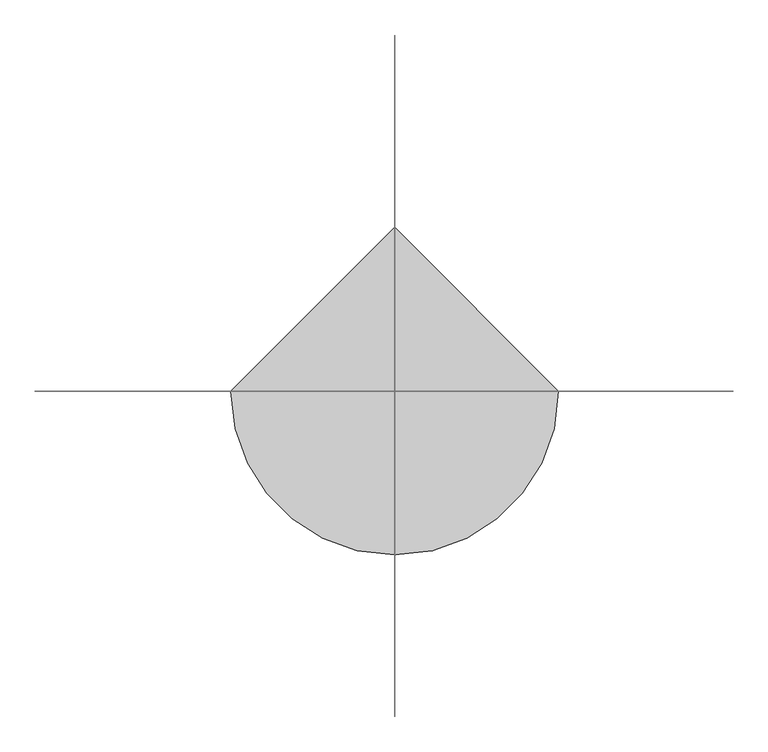
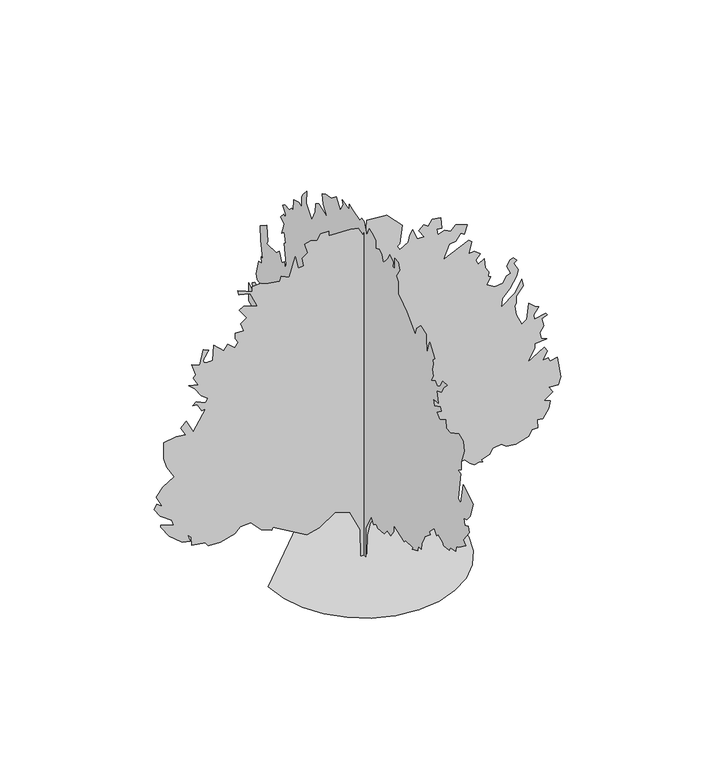
"""IFC4 building model written with IfcOpenShell, lengths in millimetres: proxy geometry, daphne 26070 : daphne 26070."""

from ifc_helpers import new_model, si_unit, origin, place, context, project, spatial, triangles, source, transform, mapped, element, save


def entourage_7462b660(model_context):
    return source(origin(), model_context, "Body", "Tessellation", [
        triangles([(-9.4573925, -3.9e-06, 72.2348623), (-36.4693492, -6.1e-06, 128.8771626), (-74.629579, -5.2e-06, 141.2324949), (-113.9485589, -1.8e-06, 114.0498972), (-145.9624841, 1e-07, 106.0463523), (-234.001251, 8e-07, 158.0691489), (-236.002001, 1.4e-06, 150.0658583), (-264.0154255, 1.9e-06, 162.0709213), (-290.0250479, 1.3e-06, 190.0833467), (-318.0387268, 2.7e-06, 188.0823242), (-332.0443036, 4.1e-06, 174.0762387), (-368.4272936, 6.4e-06, 163.6409018), (-400.0731817, 7.6e-06, 166.0726938), (-408.0767266, 7.3e-06, 176.0772612), (-442.0924192, 8.5e-06, 182.0797836), (-444.0939686, 7.2e-06, 204.089414), (-452.0975135, 7.1e-06, 212.0929589), (-446.0929381, 7.9e-06, 194.0851191), (-466.1030903, 8.6e-06, 198.0868916), (-500.1187829, 8.4e-06, 226.0990444), (-522.1279046, 7.4e-06, 258.1124609), (-522.1279046, 7.1e-06, 264.1170363), (-488.1121757, 6.3e-06, 252.1104472), (-494.1142076, 5.6e-06, 268.117537), (-522.9229142, 5.6e-06, 288.9353979), (-538.1349944, 4.9e-06, 312.1357804), (-532.1304191, 3.9e-06, 324.1423513), (-518.1248423, 3.9e-06, 314.1372934), (-534.1319321, 2.8e-06, 344.14996), (-516.6084741, 8e-07, 365.2878413), (-486.7989927, -1.6e-06, 383.4742676), (-506.1208148, -2.7e-06, 416.1818642), (-514.1243597, -3.9e-06, 442.1940482), (-514.1243597, -6.5e-06, 486.2122553), (-482.1101801, -8.1e-06, 490.2153176), (-458.099509, -9.1e-06, 488.2138046), (-470.1035728, -9.9e-06, 510.2229263), (-456.097996, -1.13e-05, 524.2284668), (-438.0893932, -1e-05, 488.2138046), (-406.0752136, -1.45e-05, 540.2355566), (-416.0802715, -1.39e-05, 538.236587), (-428.0868788, -1.46e-05, 558.2441957), (-440.0909062, -1.42e-05, 560.2457088), (-430.0883918, -1.51e-05, 568.2492537), (-406.0752136, -1.54e-05, 556.2426827), (-401.4955876, -1.62e-05, 567.0275259), (-418.0817845, -1.63e-05, 580.2533175), (-434.0888743, -1.7e-05, 604.2639522), (-450.0959641, -1.72e-05, 618.2720724), (-426.0853294, -1.79e-05, 612.2674971), (-438.0893932, -1.87e-05, 634.2791622), (-432.0873613, -1.94e-05, 642.2826708), (-442.0924192, -2.07e-05, 672.2953737), (-422.0823034, -2.11e-05, 664.2917925), (-412.0797526, -2.38e-05, 702.308004), (-398.0716687, -2.41e-05, 696.3059721), (-400.6802304, -2.38e-05, 693.2783226), (-403.212634, -2.35e-05, 690.2023476), (-405.5926123, -2.32e-05, 687.0248526), (-407.7439708, -2.29e-05, 683.6948959), (-409.5930948, -2.26e-05, 680.1642975), (-411.0637536, -2.23e-05, 676.3821882), (-412.0797526, -2.21e-05, 672.2953737), (-411.9857903, -2.19e-05, 668.7317104), (-410.3525688, -2.18e-05, 666.420369), (-407.434106, -2.18e-05, 665.1452288), (-403.4920137, -2.2e-05, 664.7033226), (-398.7777666, -2.22e-05, 664.8861603), (-393.5530128, -2.25e-05, 665.485615), (-388.0691179, -2.28e-05, 666.2907984), (-386.0676049, -2.52e-05, 706.3085592), (-360.0554572, -2.49e-05, 682.2978882), (-350.0529064, -2.62e-05, 696.3059721), (-332.0443036, -2.6e-05, 680.2988823), (-322.0392457, -2.72e-05, 692.3029461), (-330.0427906, -2.76e-05, 704.3095533), (-330.0427906, -2.84e-05, 718.3150938), (-308.0336689, -2.94e-05, 718.3150938), (-316.0372138, -3.03e-05, 740.3242155), (-301.0029389, -3.16e-05, 751.5637184), (-320.0377327, -3.24e-05, 778.340427), (-308.0336689, -3.33e-05, 784.3424589), (-274.0179581, -3.42e-05, 774.3399445), (-292.0265791, -3.57e-05, 812.356156), (-320.9191106, -3.49e-05, 820.7254852), (-324.0407587, -3.54e-05, 832.3637283), (-304.0306247, -3.58e-05, 824.3602198), (-286.0245472, -3.62e-05, 816.3566385), (-286.0245472, -3.7e-05, 830.3647951), (-265.0619096, -3.8e-05, 832.6329706), (-252.0090908, -3.82e-05, 826.3616964), (-215.9931387, -3.95e-05, 820.3596645), (-211.9913662, -4.03e-05, 832.3637283), (-191.9827583, -4.06e-05, 822.3612139), (-175.9756504, -4.43e-05, 872.3814892), (-168.7203883, -4.27e-05, 839.3385933), (-153.9660381, -4.34e-05, 840.3673096), (-157.9678106, -4.45e-05, 862.3789747), (-143.9617251, -4.57e-05, 872.3814892), (-151.9650156, -4.69e-05, 898.3936369), (-135.9581802, -4.78e-05, 902.3941195), (-119.9513447, -4.83e-05, 898.3936369), (-109.9467864, -4.96e-05, 912.3991774), (-89.9381694, -5.05e-05, 912.3991774), (-89.9381694, -4.97e-05, 900.3951862), (-32.626833, -5.21e-05, 897.7739073), (-14.3439498, -5.26e-05, 893.5625364), (-1.8993678, -5.19e-05, 872.3814892), (6.1041838, -5.31e-05, 886.3895731), (8.105045, -5.45e-05, 908.3986948), (59.627565, -5.65e-05, 903.8140182), (99.4230465, -5.58e-05, 862.5999641), (92.1418776, -5.26e-05, 814.3577053), (86.1393461, -5.21e-05, 810.3546066), (92.1418776, -5.16e-05, 798.3505428), (114.1514989, -5.33e-05, 810.3546066), (118.1578496, -5.45e-05, 827.9416145), (126.1568253, -5.56e-05, 840.3673096), (138.1621427, -5.45e-05, 812.356156), (155.7905089, -5.52e-05, 811.8684677), (142.1639151, -5.58e-05, 832.3637283), (154.1689872, -5.71e-05, 844.3703356), (166.1743046, -5.71e-05, 836.3667543), (176.1785995, -5.85e-05, 852.3739168), (198.1884842, -5.92e-05, 848.3708181), (200.188998, -5.75e-05, 818.3581879), (188.1839168, -5.71e-05, 820.3596645), (190.1846849, -5.63e-05, 804.3525747), (208.1927972, -5.74e-05, 810.3546066), (224.199887, -5.76e-05, 802.3510981), (236.20495, -5.9e-05, 816.3566385), (265.7807247, -5.96e-05, 805.7293076), (258.2140718, -5.79e-05, 782.343453), (250.2110355, -5.79e-05, 788.3454849), (236.20495, -5.62e-05, 770.3369184), (220.1978602, -5.54e-05, 768.3379126), (204.1910248, -5.26e-05, 732.3207069), (270.2206608, -5.73e-05, 762.3333372), (278.2242057, -5.71e-05, 754.3298286), (270.2206608, -5.5e-05, 724.3171257), (284.2262195, -5.57e-05, 726.318675), (300.2333274, -5.57e-05, 714.3120678), (288.2267384, -5.43e-05, 700.3065273), (294.2312955, -5.39e-05, 688.3024635), (309.737998, -5.51e-05, 697.179756), (312.8444218, -5.37e-05, 671.3504459), (322.242431, -5.33e-05, 658.2872171), (320.240918, -5.25e-05, 646.283226), (326.2454933, -5.25e-05, 642.2801273), (316.2403991, -5.1e-05, 624.2741043), (337.7847236, -5.12e-05, 610.9797123), (358.2596729, -5.23e-05, 614.2690464), (368.2621874, -5.37e-05, 630.2761362), (378.0386619, -5.44e-05, 634.7135107), (368.2621874, -5.52e-05, 656.2882839), (376.2657323, -5.64e-05, 670.2938244), (384.2692772, -5.7e-05, 674.2943069), (394.2743714, -5.68e-05, 664.2917925), (386.2708265, -5.61e-05, 658.2872171), (398.1707179, -5.54e-05, 637.1290609), (394.2743714, -5.43e-05, 622.272555), (376.2657323, -5.17e-05, 592.2598884), (356.2581599, -4.97e-05, 572.2497725), (354.2566106, -4.83e-05, 550.2406508), (388.2723395, -5.13e-05, 576.2527986), (406.2783989, -5.4e-05, 608.2669782), (410.2814612, -5.3e-05, 588.2568624), (392.2728221, -5.09e-05, 566.2477407), (392.2728221, -4.98e-05, 548.2391015), (388.2723395, -4.93e-05, 542.2371059), (392.2728221, -4.79e-05, 516.2249219), (406.2783989, -4.67e-05, 486.2122553), (419.6692966, -4.79e-05, 495.1530613), (424.2870017, -5.05e-05, 536.235074), (440.2941278, -5.04e-05, 522.2294972), (450.2991858, -5.06e-05, 518.2264712), (437.047996, -4.89e-05, 500.1924339), (438.2925785, -4.83e-05, 488.2138046), (468.3077886, -4.99e-05, 494.2158002), (472.3083075, -4.97e-05, 488.2138046), (458.3027307, -4.88e-05, 482.2117727), (462.5902596, -4.78e-05, 462.3895815), (452.3006988, -4.64e-05, 446.1945308), (456.3012177, -4.56e-05, 430.187441), (470.3067581, -4.58e-05, 424.1854091), (440.2941278, -4.43e-05, 420.1849265), (440.2941278, -4.36e-05, 408.1783193), (420.2865191, -4.08e-05, 376.1641397), (464.3047626, -4.43e-05, 402.1762874), (472.3083075, -4.39e-05, 390.1697165), (460.3017002, -4.21e-05, 368.1605947), (474.3098205, -4.28e-05, 370.1621078), (478.3103394, -4.24e-05, 360.1570498), (498.3204552, -4.35e-05, 364.1600759), (506.3240001, -4.05e-05, 308.1352615), (500.3194247, -3.9e-05, 288.1251276), (476.3113335, -3.81e-05, 290.1266587), (486.3138843, -3.76e-05, 274.1195508), (464.3047626, -3.57e-05, 258.1124609), (480.3118524, -3.6e-05, 252.1104472), (476.3113335, -3.47e-05, 232.1015668), (460.3017002, -3.26e-05, 210.0919546), (446.2961234, -3.22e-05, 212.0929589), (448.2976727, -3.09e-05, 190.0833467), (432.2905829, -3.02e-05, 190.0833467), (424.2870017, -2.89e-05, 174.0762387), (391.7419679, -2.69e-05, 164.3614974), (366.2632178, -2.6e-05, 168.0737163), (354.2566106, -2.61e-05, 178.0780111), (332.2474889, -2.49e-05, 174.0762387), (323.8020015, -2.37e-05, 160.8723026), (302.2348404, -2.24e-05, 154.0673764), (306.2353412, -2.21e-05, 146.0640859), (298.2317963, -2.2e-05, 150.0658583), (284.2262195, -2.11e-05, 146.0640859), (272.2196304, -2.11e-05, 154.0673764), (260.2155848, -2.14e-05, 168.0737163), (240.2064682, -2.03e-05, 164.0719438), (236.8051496, -1.96e-05, 155.3752181), (196.1874799, -1.67e-05, 136.0595276), (196.1874799, -1.6e-05, 124.0544646), (162.1725321, -1.36e-05, 110.0481247), (162.1725321, -1.4e-05, 116.0509106), (138.1618883, -1.27e-05, 112.0491381), (106.7192036, -1.23e-05, 127.7984221), (83.214788, -1.13e-05, 128.4156446), (38.7434109, -8e-06, 104.983363), (17.3291135, -5.6e-06, 81.0641653), (9.1189377, -3.5e-06, 51.8726831), (8.1050195, -4e-07, 0.0), (-7.9020227, 3e-07, 7e-07), (-244.9072532, 0.0, 4.54e-05), (-238.4327937, -56.1165193, 4.18e-05), (-219.9933851, -107.6506239, 3.79e-05), (-191.0655541, -153.1257915, 3.39e-05), (-153.1257915, -191.0655541, 3e-05), (-107.6506239, -219.9933851, 2.63e-05), (-56.1165193, -238.4327937, 2.29e-05), (1.14e-05, -244.9072532, 2.01e-05), (56.1165193, -238.4327937, 1.8e-05), (107.6506239, -219.9933851, 5.12e-05), (153.1257915, -191.0655541, 5.1e-05), (191.0655541, -153.1257915, 5.16e-05), (219.9933851, -107.6506239, 1.87e-05), (238.4327937, -56.1165193, 2.09e-05), (244.9072532, 2.14e-05, 2.4e-05), (-3.16e-05, 244.9072532, 4.93e-05), (-1e-06, -8.7682648, 19.1210077), (-2.7e-06, -9.3654196, 78.8180451), (-6.1e-06, -33.2534526, 124.0544646), (-5.1e-06, -45.2590243, 110.0481247), (-5.2e-06, -55.2633328, 118.0516787), (-5.8e-06, -63.2666234, 112.0491381), (-6.9e-06, -91.2787853, 114.0498972), (-9e-06, -105.285116, 130.0569961), (-9.8e-06, -121.2919515, 126.0552236), (-9.6e-06, -133.2972779, 144.0630725), (-1.09e-05, -133.2972779, 162.0709213), (-1.16e-05, -181.318293, 146.0640859), (-1.37e-05, -187.3210879, 152.0666174), (-1.51e-05, -221.3357813, 154.0676308), (-1.31e-05, -215.3334951, 146.0640859), (-1.58e-05, -241.3446436, 158.0694032), (-1.53e-05, -243.3454117, 172.0754887), (-1.59e-05, -257.3504617, 172.0754887), (-1.75e-05, -259.3519928, 188.0825785), (-1.71e-05, -267.3555377, 204.089414), (-1.9e-05, -271.3585819, 214.0939814), (-1.92e-05, -297.3682044, 236.1036118), (-2.09e-05, -291.3661725, 240.1051299), (-2.09e-05, -315.3768253, 264.1170363), (-2.19e-05, -325.3818832, 250.1096791), (-2.19e-05, -331.3839151, 256.1134914), (-2.32e-05, -351.394031, 248.1086748), (-2.37e-05, -357.3960629, 242.1061342), (-2.46e-05, -381.4066976, 244.1069023), (-2.44e-05, -385.4072165, 254.1119602), (-2.53e-05, -409.4178512, 258.1124609), (-2.69e-05, -411.4193642, 272.1180377), (-2.71e-05, -423.423428, 278.1225949), (-2.96e-05, -455.4376076, 302.1332478), (-2.88e-05, -443.4335438, 310.1367745), (-3.05e-05, -469.4457278, 346.151473), (-3.18e-05, -465.4426655, 360.1570498), (-3.14e-05, -449.4355757, 354.1550179), (-3.05e-05, -445.4350931, 370.1621078), (-3.1e-05, -459.4406336, 374.1651701), (-3.29e-05, -474.5104623, 393.7968206), (-3.38e-05, -487.4517872, 434.1905033), (-3.29e-05, -443.4335438, 460.202651), (-3.07e-05, -433.4284859, 404.1778367), (-3e-05, -421.4244221, 408.1783193), (-3.36e-05, -431.6073034, 483.065209), (-3.29e-05, -419.4229091, 486.2122553), (-3.32e-05, -435.4299989, 496.2173495), (-3.43e-05, -435.4299989, 518.2264712), (-3.54e-05, -447.4340627, 554.2436769), (-3.64e-05, -443.4335438, 578.2543116), (-3.73e-05, -423.423428, 586.2578565), (-3.43e-05, -384.7290238, 566.6439737), (-3.35e-05, -367.3985773, 568.2492537), (-3.46e-05, -365.3996078, 590.2583754), (-3.2e-05, -339.38746, 574.2512856), (-3.09e-05, -325.3818832, 586.2578565), (-3.33e-05, -345.3894919, 600.2634333), (-3.26e-05, -341.388973, 610.2684912), (-3.2e-05, -313.375276, 596.2604073), (-3.12e-05, -309.3747934, 612.2674971), (-3.2e-05, -331.3839151, 614.2690464), (-3.26e-05, -324.6503509, 643.5704556), (-3.53e-05, -345.3894919, 652.2852579), (-3.49e-05, -357.3960629, 672.2953737), (-3.71e-05, -373.4031527, 688.3024635), (-3.62e-05, -351.394031, 686.3009142), (-3.44e-05, -341.388973, 668.2923477), (-3.42e-05, -327.3833962, 658.2897606), (-3.34e-05, -319.3798513, 668.2923477), (-3.31e-05, -301.3712485, 658.2897606), (-3.49e-05, -309.3747934, 674.2943069), (-3.4e-05, -305.3717311, 690.3013968), (-3.56e-05, -309.3747934, 706.3085592), (-3.5e-05, -307.3732804, 718.3150938), (-3.51e-05, -317.3783383, 726.318675), (-3.49e-05, -295.3692166, 758.3328547), (-3.52e-05, -289.3646595, 744.3272415), (-3.4e-05, -281.3610964, 716.3136171), (-3.58e-05, -279.3621268, 770.3369184), (-3.44e-05, -255.3514921, 778.340427), (-3.23e-05, -237.3428711, 760.334404), (-3.28e-05, -229.3393262, 740.3242155), (-3.11e-05, -209.330464, 760.334404), (-3.16e-05, -191.322606, 778.340427), (-3.05e-05, -177.3165205, 790.3470343), (-3.1e-05, -153.3061402, 804.3525747), (-3.17e-05, -153.3061402, 836.3667543), (-3.08e-05, -145.3025953, 848.3708181), (-3.26e-05, -161.3094307, 872.3814892), (-3.37e-05, -155.087445, 890.4942644), (-3.3e-05, -138.6373771, 891.588965), (-3.2e-05, -138.6373771, 863.4050749), (-3.17e-05, -129.7796238, 863.4050749), (-3.12e-05, -131.2962645, 876.3845152), (-3.22e-05, -115.28942, 886.3895731), (-3.04e-05, -107.2858751, 870.3824833), (-2.83e-05, -87.2770128, 848.3708181), (-2.94e-05, -81.2744813, 866.3794573), (-2.85e-05, -69.2691594, 874.3829659), (-2.82e-05, -53.2620651, 866.3794573), (-2.94e-05, -53.2620651, 888.388579), (-2.86e-05, -42.0070608, 894.8096987), (-2.75e-05, -25.2500576, 902.3966629), (-2.59e-05, -13.2446369, 878.3860645), (-2.63e-05, -3.2402807, 908.3986948), (-2.57e-05, 8.7649884, 910.4002441), (-2.58e-05, 16.768535, 900.3951862), (-2.39e-05, 50.7832783, 910.4002441), (-2.52e-05, 64.7893547, 914.4007267), (-2.37e-05, 64.7893547, 900.3951862), (-2.2e-05, 94.8025255, 908.3986948), (-2.26e-05, 90.8010074, 898.3936369), (-2.09e-05, 104.8068295, 874.3829659), (-2.11e-05, 122.8149417, 900.3951862), (-1.88e-05, 144.7590329, 883.3085838), (-1.79e-05, 169.2642141, 879.2750364), (-1.76e-05, 184.8420423, 870.3824833), (-1.68e-05, 179.1326343, 845.1882362), (-1.65e-05, 162.8324119, 820.3596645), (-1.63e-05, 200.8491321, 834.3652777), (-1.4e-05, 212.8544495, 826.3616964), (-1.49e-05, 216.8562219, 802.3510981), (-1.34e-05, 230.8623074, 772.3383951), (-1.32e-05, 254.871416, 802.3510981), (-1.4e-05, 252.8719378, 836.3667543), (-1.19e-05, 270.8810493, 816.3566385), (-1.21e-05, 276.8830812, 806.3541241), (-1.12e-05, 276.8830812, 778.340427), (-1.04e-05, 288.8871268, 784.3450024), (-9.7e-06, 310.8962485, 778.340427), (-8.7e-06, 314.8992745, 746.3262474), (-8.4e-06, 320.9013064, 748.3277967), (-6.3e-06, 330.9064007, 738.3227388), (-5.3e-06, 350.913973, 740.3242155), (-5.2e-06, 360.919031, 732.3207069), (-6.5e-06, 346.9134905, 716.3136171), (-4.7e-06, 348.9150035, 706.3085592), (-4.2e-06, 356.9185484, 710.3115852), (-4.3e-06, 368.9226122, 696.3059721), (-5.4e-06, 354.9170354, 684.2994375), (-4.1e-06, 364.9220933, 654.2867346), (-4.2e-06, 354.9170354, 662.2903158), (-3.5e-06, 346.9134905, 638.2796448), (-3.4e-06, 354.9170354, 632.2776129), (-1.8e-06, 344.9119411, 580.2533175), (-2.2e-06, 348.9150035, 568.2492537), (-1.3e-06, 354.9170354, 582.2548305), (-1.2e-06, 365.0364032, 574.0988966), (-1.8e-06, 376.9261571, 598.2619203), (4e-07, 388.932728, 586.2578565), (2.2e-06, 432.9509714, 584.2563435), (2.4e-06, 426.9489395, 594.2614014), (1e-07, 432.9509714, 634.2791622), (2.7e-06, 460.962125, 616.2705231), (3.1e-06, 458.9631191, 578.2543116), (5e-06, 448.9580612, 534.233561), (5.4e-06, 456.9616061, 534.233561), (4.5e-06, 453.2786187, 518.6607834), (5e-06, 466.966664, 516.2274653), (8e-06, 478.9707278, 474.2082278), (7.2e-06, 474.9702089, 460.202651), (6.5e-06, 460.962125, 458.201138), (7.6e-06, 458.9631191, 436.1920163), (9.3e-06, 484.9727597, 448.1960438), (9.4e-06, 495.8998544, 440.6471586), (1.04e-05, 490.9772987, 418.1833772), (9.7e-06, 512.9864204, 430.187441), (1.18e-05, 512.9864204, 380.167202), (9.6e-06, 476.9692148, 366.1616252), (1.23e-05, 498.9808436, 356.156531), (1.21e-05, 504.9828755, 346.151473), (1.23e-05, 478.9707278, 328.1428702), (1.17e-05, 462.963638, 330.1443832), (1.21e-05, 484.9727597, 316.1388064), (1.23e-05, 514.7745744, 340.233266), (1.35e-05, 520.9899653, 312.1357804), (1.38e-05, 508.9833944, 282.1231138), (1.52e-05, 530.9950596, 292.1281717), (1.67e-05, 532.7171565, 276.4538196), (1.52e-05, 513.8677983, 260.1292346), (1.52e-05, 504.9828755, 270.11905), (1.29e-05, 491.4116472, 278.5442443), (1.42e-05, 500.9798495, 300.1317166), (1.21e-05, 492.9763046, 308.1352615), (1.3e-05, 481.8053658, 291.1223283), (1.34e-05, 462.963638, 270.11905), (1.3e-05, 470.9671829, 252.1104472), (1.42e-05, 484.9727597, 266.1160058), (1.4e-05, 490.9772987, 256.1134914), (1.53e-05, 488.9757857, 238.1043617), (1.35e-05, 462.963638, 224.0982762), (1.52e-05, 472.9686959, 202.088664), (1.48e-05, 492.9763046, 222.0972719), (1.65e-05, 493.9364204, 210.9735868), (1.65e-05, 480.9722408, 176.0772612), (1.56e-05, 460.962125, 176.0772612), (1.7e-05, 462.963638, 156.0683989), (1.44e-05, 448.9580612, 160.0701714), (1.53e-05, 434.1422141, 145.3175835), (1.52e-05, 426.9489395, 150.0658583), (1.32e-05, 388.932728, 142.0623134), (1.26e-05, 374.9246078, 144.0630725), (1.31e-05, 378.9276701, 150.0658583), (1.21e-05, 350.913973, 156.0683989), (1.15e-05, 348.9150035, 144.0630725), (1.1e-05, 338.9099456, 142.0623134), (1.02e-05, 326.9033383, 136.0595276), (7.2e-06, 286.8856138, 158.0691489), (8.6e-06, 278.8845942, 148.0648449), (6.5e-06, 264.0916381, 164.6055958), (5.2e-06, 240.8666204, 158.0691489), (3.7e-06, 204.8506502, 158.0694032), (3.3e-06, 166.8341844, 138.060541), (3e-06, 170.8359568, 128.056237), (4.5e-06, 158.8306395, 124.0544646), (2.7e-06, 158.8306395, 132.0580095), (2e-06, 144.8243087, 130.0569961), (1.3e-06, 120.8141827, 138.060541), (-1e-06, 101.9528885, 154.2177488), (-2.5e-06, 36.7154756, 135.157575), (-1.1e-06, 12.638517, 93.3765678), (1.1e-06, 8.7649628, 3.52e-05), (3e-07, -9.2429405, 3.42e-05)], [[48, 49, 50], [94, 95, 96], [184, 185, 186], [212, 213, 214], [165, 166, 167], [165, 167, 168], [42, 43, 44], [52, 53, 54], [70, 71, 72], [42, 44, 45], [85, 86, 87], [84, 85, 87], [84, 87, 88], [41, 42, 45], [40, 41, 45], [173, 174, 175], [117, 118, 119], [17, 18, 19], [116, 117, 119], [144, 145, 146], [221, 222, 223], [21, 22, 23], [20, 21, 23], [132, 133, 134], [131, 132, 134], [130, 131, 134], [37, 38, 39], [36, 37, 39], [55, 56, 57], [164, 165, 168], [164, 168, 169], [164, 169, 170], [175, 176, 177], [173, 175, 177], [125, 126, 127], [179, 180, 181], [178, 179, 181], [173, 177, 178], [130, 134, 135], [130, 135, 136], [124, 125, 127], [123, 124, 127], [6, 7, 8], [26, 27, 28], [25, 26, 28], [80, 81, 82], [80, 82, 83], [157, 158, 159], [156, 157, 159], [155, 156, 159], [154, 155, 159], [154, 159, 160], [154, 160, 161], [92, 93, 94], [72, 73, 74], [203, 204, 205], [141, 142, 143], [193, 194, 195], [99, 100, 101], [55, 57, 58], [103, 104, 105], [76, 77, 78], [75, 76, 78], [109, 110, 111], [140, 141, 143], [99, 101, 102], [229, 230, 231], [229, 231, 1], [228, 229, 1], [188, 189, 190], [188, 190, 191], [197, 198, 199], [102, 103, 105], [148, 149, 150], [17, 19, 20], [17, 20, 23], [88, 89, 90], [154, 161, 162], [153, 154, 162], [152, 153, 162], [152, 162, 163], [151, 152, 163], [33, 34, 35], [228, 1, 2], [227, 228, 2], [83, 84, 88], [199, 200, 201], [47, 48, 50], [121, 122, 123], [120, 121, 123], [120, 123, 127], [120, 127, 128], [195, 196, 197], [193, 195, 197], [220, 221, 223], [191, 192, 193], [14, 15, 16], [78, 79, 80], [55, 58, 59], [54, 55, 59], [54, 59, 60], [54, 60, 61], [54, 61, 62], [54, 62, 63], [54, 63, 64], [54, 64, 65], [183, 184, 186], [129, 130, 136], [128, 129, 136], [137, 138, 139], [137, 139, 140], [83, 88, 90], [83, 90, 91], [83, 91, 92], [164, 170, 171], [28, 29, 30], [191, 193, 197], [188, 191, 197], [50, 51, 52], [24, 25, 28], [97, 98, 99], [109, 111, 112], [109, 112, 113], [109, 113, 114], [108, 109, 114], [128, 136, 137], [120, 128, 137], [201, 202, 203], [199, 201, 203], [178, 181, 182], [178, 182, 183], [33, 35, 36], [32, 33, 36], [31, 32, 36], [31, 36, 39], [119, 120, 137], [28, 30, 31], [52, 54, 65], [52, 65, 66], [50, 52, 66], [50, 66, 67], [50, 67, 68], [50, 68, 69], [116, 119, 137], [115, 116, 137], [172, 173, 178], [172, 178, 183], [172, 183, 186], [188, 197, 199], [24, 28, 31], [50, 69, 70], [214, 215, 216], [212, 214, 216], [212, 216, 217], [47, 50, 70], [46, 47, 70], [46, 70, 72], [46, 72, 74], [12, 13, 14], [205, 206, 207], [106, 107, 108], [137, 140, 143], [226, 227, 2], [146, 147, 148], [4, 5, 6], [3, 4, 6], [99, 102, 105], [97, 99, 105], [97, 105, 106], [97, 106, 108], [97, 108, 114], [97, 114, 115], [218, 219, 220], [137, 143, 144], [188, 199, 203], [188, 203, 205], [188, 205, 207], [188, 207, 208], [188, 208, 209], [188, 209, 210], [210, 211, 212], [210, 212, 217], [188, 210, 217], [188, 217, 218], [6, 8, 9], [78, 80, 83], [223, 224, 225], [220, 223, 225], [83, 92, 94], [11, 12, 14], [10, 11, 14], [10, 14, 16], [10, 16, 17], [10, 17, 23], [10, 23, 24], [10, 24, 31], [10, 31, 39], [9, 10, 39], [9, 39, 40], [6, 9, 40], [3, 6, 40], [3, 40, 45], [3, 45, 46], [3, 46, 74], [3, 74, 75], [3, 75, 78], [3, 78, 83], [3, 83, 94], [3, 94, 96], [3, 96, 97], [3, 97, 115], [3, 115, 137], [2, 3, 137], [226, 2, 137], [226, 137, 144], [226, 144, 146], [226, 146, 148], [226, 148, 150], [225, 226, 150], [220, 225, 150], [218, 220, 150], [188, 218, 150], [150, 151, 163], [150, 163, 164], [188, 150, 164], [188, 164, 171], [188, 171, 172], [188, 172, 186], [187, 188, 186], [246, 247, 232], [245, 246, 232], [245, 232, 233], [244, 245, 233], [244, 233, 234], [244, 234, 235], [243, 244, 235], [242, 243, 235], [242, 235, 236], [242, 236, 237], [242, 237, 238], [242, 238, 239], [242, 239, 240], [242, 240, 241], [261, 262, 263], [388, 389, 390], [372, 373, 374], [312, 313, 314], [440, 441, 442], [440, 442, 443], [312, 314, 315], [311, 312, 315], [358, 359, 360], [323, 324, 325], [414, 415, 416], [422, 423, 424], [301, 302, 303], [449, 450, 451], [400, 401, 402], [400, 402, 403], [399, 400, 403], [444, 445, 446], [311, 315, 316], [310, 311, 316], [289, 290, 291], [288, 289, 291], [287, 288, 291], [286, 287, 291], [280, 281, 282], [396, 397, 398], [322, 323, 325], [322, 325, 326], [462, 463, 464], [461, 462, 464], [425, 426, 427], [425, 427, 428], [425, 428, 429], [440, 443, 444], [268, 269, 270], [356, 357, 358], [394, 395, 396], [435, 436, 437], [435, 437, 438], [435, 438, 439], [425, 429, 430], [425, 430, 431], [424, 425, 431], [404, 405, 406], [372, 374, 375], [372, 375, 376], [456, 457, 458], [271, 272, 273], [371, 372, 376], [414, 416, 417], [308, 309, 310], [342, 343, 344], [341, 342, 344], [305, 306, 307], [304, 305, 307], [283, 284, 285], [282, 283, 285], [338, 339, 340], [337, 338, 340], [336, 337, 340], [361, 362, 363], [382, 383, 384], [381, 382, 384], [470, 471, 248], [469, 470, 248], [469, 248, 249], [469, 249, 250], [468, 469, 250], [386, 387, 388], [385, 386, 388], [399, 403, 404], [250, 251, 252], [350, 351, 352], [418, 419, 420], [417, 418, 420], [417, 420, 421], [321, 322, 326], [320, 321, 326], [292, 293, 294], [264, 265, 266], [316, 317, 318], [310, 316, 318], [308, 310, 318], [446, 447, 448], [424, 431, 432], [422, 424, 432], [422, 432, 433], [364, 365, 366], [277, 278, 279], [261, 263, 264], [255, 256, 257], [398, 399, 404], [326, 327, 328], [326, 328, 329], [326, 329, 330], [452, 453, 454], [396, 398, 404], [412, 413, 414], [411, 412, 414], [411, 414, 417], [377, 378, 379], [376, 377, 379], [336, 340, 341], [408, 409, 410], [341, 344, 345], [421, 422, 433], [421, 433, 434], [363, 364, 366], [363, 366, 367], [361, 363, 367], [407, 408, 410], [406, 407, 410], [391, 392, 393], [336, 341, 345], [255, 257, 258], [258, 259, 260], [379, 380, 381], [275, 276, 277], [274, 275, 277], [352, 353, 354], [352, 354, 355], [348, 349, 350], [348, 350, 352], [346, 347, 348], [345, 346, 348], [297, 298, 299], [297, 299, 300], [296, 297, 300], [294, 295, 296], [294, 296, 300], [294, 300, 301], [335, 336, 345], [334, 335, 345], [454, 455, 456], [452, 454, 456], [358, 360, 361], [367, 368, 369], [367, 369, 370], [286, 291, 292], [355, 356, 358], [448, 449, 451], [439, 440, 444], [396, 404, 406], [394, 396, 406], [394, 406, 410], [394, 410, 411], [371, 376, 379], [367, 370, 371], [294, 301, 303], [253, 254, 255], [252, 253, 255], [292, 294, 303], [318, 319, 320], [318, 320, 326], [318, 326, 330], [434, 435, 439], [352, 355, 358], [352, 358, 361], [352, 361, 367], [260, 261, 264], [411, 417, 421], [394, 411, 421], [252, 255, 258], [250, 252, 258], [348, 352, 367], [345, 348, 367], [334, 345, 367], [334, 367, 371], [333, 334, 371], [332, 333, 371], [331, 332, 371], [330, 331, 371], [318, 330, 371], [308, 318, 371], [307, 308, 371], [307, 371, 379], [307, 379, 381], [307, 381, 384], [307, 384, 385], [307, 385, 388], [307, 388, 390], [307, 390, 391], [307, 391, 393], [307, 393, 394], [307, 394, 421], [307, 421, 434], [307, 434, 439], [307, 439, 444], [307, 444, 446], [307, 446, 448], [307, 448, 451], [307, 451, 452], [307, 452, 456], [307, 456, 458], [307, 458, 459], [307, 459, 460], [307, 460, 461], [307, 461, 464], [307, 464, 465], [307, 465, 466], [307, 466, 467], [307, 467, 468], [307, 468, 250], [307, 250, 258], [304, 307, 258], [303, 304, 258], [292, 303, 258], [292, 258, 260], [273, 274, 277], [273, 277, 279], [271, 273, 279], [279, 280, 282], [271, 279, 282], [271, 282, 285], [271, 285, 286], [271, 286, 292], [271, 292, 260], [270, 271, 260], [268, 270, 260], [268, 260, 264], [268, 264, 266], [268, 266, 267]], closed=False),
    ])


if __name__ == "__main__":
    model = new_model("IFC4")
    model_context = context("Model", 3, world=origin())
    ifc_project = project(units=[si_unit("LENGTHUNIT", "METRE", prefix="MILLI")], contexts=[model_context])
    site = spatial("IfcSite", under=ifc_project)
    building = spatial("IfcBuilding", under=site)
    placement = place(None, origin())
    entourage_shape = entourage_7462b660(model_context)
    element("IfcBuildingElementProxy", 1, Name="daphne 26070 : daphne 26070", ObjectType="daphne 26070 : daphne 26070", at=placement, inside=building, context=model_context, shape_type="MappedRepresentation", body=[
        mapped(entourage_shape, transform((0.0, 0.0, 0.0), x_axis=(1.0, 0.0, 0.0), y_axis=(0.0, 1.0, 0.0), z_axis=(0.0, 0.0, 1.0))),
    ])
    save(model, "model.ifc")

# Revit data of these elements
# Type "daphne 26070 : daphne 26070"
#   built-in parameter 1005195 = "RPC-16-FUMB-EMQ0-U9RG-4000-ST1L-LVER-AU"
#   Height = 0
